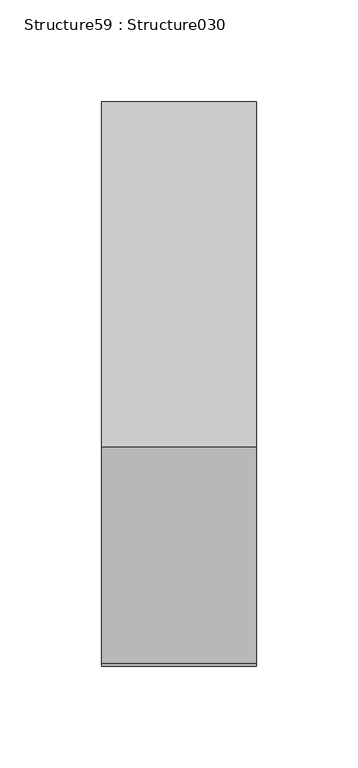
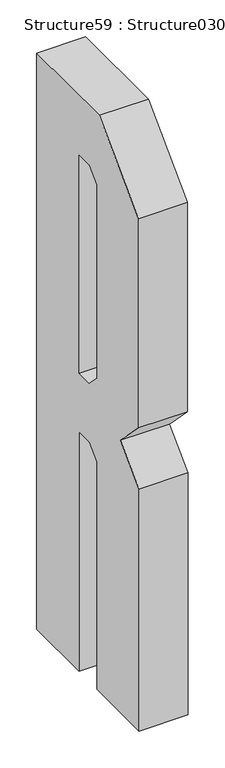
"""IFC4 building model written with IfcOpenShell, lengths in millimetres: proxy geometry, Structure59 : Structure030."""

from ifc_helpers import new_model, si_unit, frame, origin, place, context, project, spatial, polyline, outline, extrude, source, transform, mapped, element, save


def structure59_structure030_2b751848(model_context):
    return source(origin(), model_context, "Body", "SweptSolid", [
        extrude(outline(polyline([(282115.882627, 4374.3842509), (282221.9403707, 4480.4419946), (282391.9125114, 4480.4419946), (282391.9125114, 3528.5825142), (282277.702826, 3528.5825142), (282277.702826, 3924.2892507), (282249.1433195, 3924.2892507), (282228.7452015, 3903.8911328), (282228.7452015, 3528.5825142), (282114.5096949, 3528.5825142), (282114.5096949, 3928.3570344), (282164.8308046, 3978.6781441), (282115.882627, 4028.9992538), (282115.882627, 4374.3842509)]), holes=[polyline([(282277.702826, 4020.827159), (282277.702826, 4381.1897115), (282250.4992474, 4381.1897115), (282230.1011294, 4360.7915935), (282230.1011294, 4041.2277961), (282250.5017665, 4020.827159), (282277.702826, 4020.827159)])]), frame((-59031.6926606, 0.0, 0.0), z_axis=(1.0, 0.0, 0.0), x_axis=(0.0, 1.0, 0.0)), (0.0, 0.0, 1.0), 76.2),
    ])


if __name__ == "__main__":
    model = new_model("IFC4")
    model_context = context("Model", 3, world=origin())
    ifc_project = project(units=[si_unit("LENGTHUNIT", "METRE", prefix="MILLI")], contexts=[model_context])
    site = spatial("IfcSite", under=ifc_project)
    building = spatial("IfcBuilding", under=site)
    placement = place(None, origin())
    structure59_structure030_shape = structure59_structure030_2b751848(model_context)
    element("IfcBuildingElementProxy", 1, Name="Structure59 : Structure030", ObjectType="Structure59 : Structure030", at=placement, inside=building, context=model_context, shape_type="MappedRepresentation", body=[
        mapped(structure59_structure030_shape, transform((0.0, 0.0, 0.0), x_axis=(1.0, 0.0, 0.0), y_axis=(0.0, 1.0, 0.0), z_axis=(0.0, 0.0, 1.0))),
    ])
    save(model, "model.ifc")

# Revit data of these elements
# Type "Structure59 : Structure030"
#   NameOverride = "Structure030"
# Element 1 (IfcBuildingElementProxy, "Structure59 : Structure030")
#   Materials on its faces: "BRUSHED ALUM. LETTERING"
# Materials
#   "BRUSHED ALUM. LETTERING": class "Unassigned", colour RGB 169 181 186, transparency 0, Cost = 0
